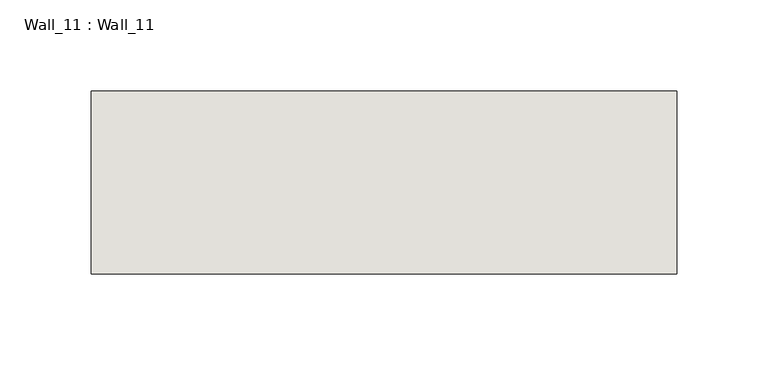
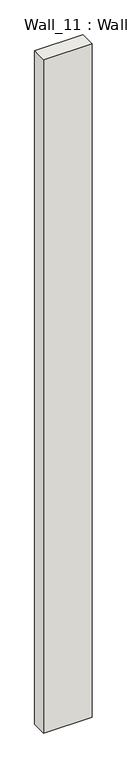
"""IFC4 building model written with IfcOpenShell, lengths in millimetres: wall geometry, Wall_11 : Wall_11."""

from ifc_helpers import new_model, si_unit, origin, origin_with_axes, place, context, project, spatial, polyline, outline, extrude, source, transform, mapped, element, save


def wall_11_wall_11_b3d456f5(model_context):
    return source(origin(), model_context, "Body", "SweptSolid", [
        extrude(outline(polyline([(4800.0, 7530.0), (4480.0, 7530.0), (4480.0, 7630.0), (4800.0, 7630.0), (4800.0, 7530.0)])), origin_with_axes(), (0.0, 0.0, 1.0), 4700.0),
    ])


if __name__ == "__main__":
    model = new_model("IFC4")
    model_context = context("Model", 3, world=origin())
    ifc_project = project(units=[si_unit("LENGTHUNIT", "METRE", prefix="MILLI")], contexts=[model_context])
    site = spatial("IfcSite", under=ifc_project)
    building = spatial("IfcBuilding", under=site)
    placement = place(None, origin())
    wall_11_wall_11_shape = wall_11_wall_11_b3d456f5(model_context)
    element("IfcWall", 1, ObjectType="Wall_11 : Wall_11", at=placement, inside=building, context=model_context, shape_type="MappedRepresentation", body=[
        mapped(wall_11_wall_11_shape, transform((0.0, 0.0, 0.0), x_axis=(1.0, 0.0, 0.0), y_axis=(0.0, 1.0, 0.0), z_axis=(0.0, 0.0, 1.0))),
    ])
    save(model, "model.ifc")

# Revit data of these elements
# Type "Wall_11 : Wall_11"
#   NameOverride = "Wall_11"
# Element 1 (IfcWall, "Wall_11 : Wall_11")
#   Materials on its faces: "IfcSurfaceStyle #33"
# Materials
#   "IfcSurfaceStyle #33": class "Unassigned", colour RGB 214 214 214, transparency 0
